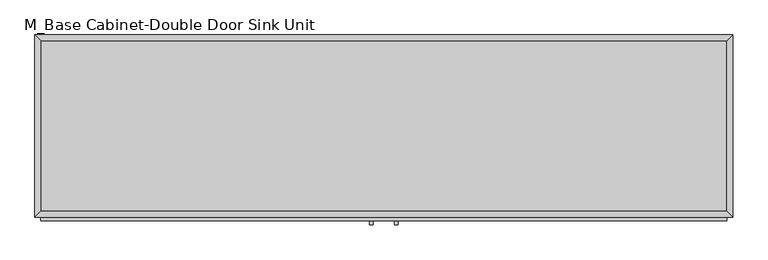
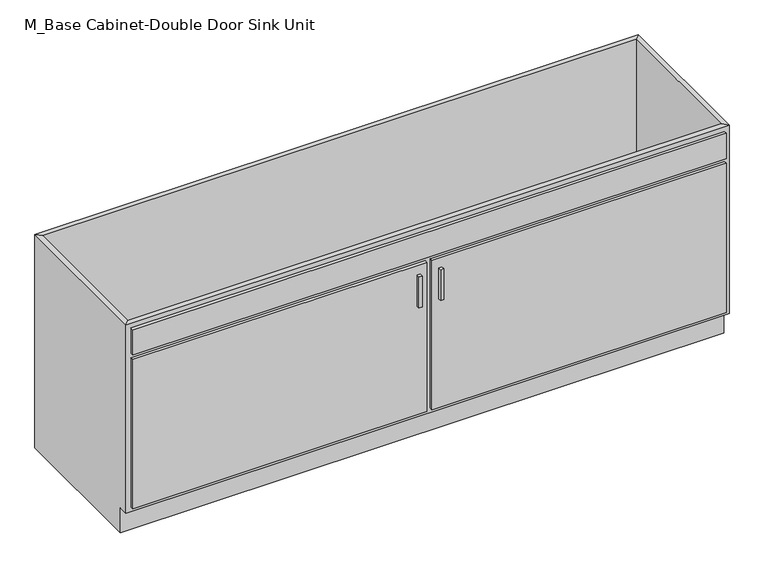
"""IFC4 building model written with IfcOpenShell, lengths in millimetres: furniture geometry, M_Base Cabinet-Double Door Sink Unit : UEBLEE."""

import ifcopenshell
import ifcopenshell.guid

model = None  # the IFC model being written
_history = None  # IfcOwnerHistory: only IFC2X3 demands one
_inside = {}  # id of a spatial element -> (the spatial element, [elements in it])
_under = {}  # id of a project, library or spatial element -> (it, [spatial elements below it])
_declared = {}  # id of a project -> (the project, [libraries it declares])
_typed = {}  # id of a type object -> (the type object, [elements of that type])
_made_of = {}  # id of a material, layer set ... -> (it, [elements and type objects made of it])


def new_model(schema):
    """Start an empty IFC model of exactly this schema.

    Asked for "IFC4X3", IfcOpenShell would pick the latest addendum, in which some entities
    have other attributes; the version numbers below select the first issue.
    IFC2X3 requires an IfcOwnerHistory on every rooted entity: one is made here for all.
    """
    global model, _history
    if schema == "IFC4X3":
        model = ifcopenshell.file(schema_version=(4, 3, 0, 0))
    else:
        model = ifcopenshell.file(schema=schema)
    _inside.clear()
    _under.clear()
    _declared.clear()
    _typed.clear()
    _made_of.clear()
    _history = None
    if model.schema == "IFC2X3":
        org = make("IfcOrganization", Name="unknown")
        user = make(
            "IfcPersonAndOrganization",
            ThePerson=make("IfcPerson", FamilyName="unknown"),
            TheOrganization=org,
        )
        app = make(
            "IfcApplication",
            ApplicationDeveloper=org,
            Version="unknown",
            ApplicationFullName="unknown",
            ApplicationIdentifier="unknown",
        )
        _history = make(
            "IfcOwnerHistory",
            OwningUser=user,
            OwningApplication=app,
            ChangeAction="ADDED",
            CreationDate=0,
        )
    return model


def make(cls, **values):
    """One entity of the class cls with the attributes given. An attribute that is None is left unset."""
    return model.create_entity(
        cls, **{name: value for name, value in values.items() if value is not None}
    )


def rooted(cls, **values):
    """An entity with a GlobalId (a new one), such as an element, a storey or a relation."""
    return make(cls, GlobalId=ifcopenshell.guid.new(), OwnerHistory=_history, **values)


def si_unit(unit_type, name, prefix=None):
    """IfcSIUnit, for example si_unit("LENGTHUNIT", "METRE", prefix="MILLI")."""
    return make("IfcSIUnit", UnitType=unit_type, Prefix=prefix, Name=name)


def assignment(units):
    """IfcUnitAssignment: the units of a project."""
    return None if units is None else make("IfcUnitAssignment", Units=units)


def point(xyz):
    """IfcCartesianPoint."""
    return None if xyz is None else make("IfcCartesianPoint", Coordinates=xyz)


def direction(xyz):
    """IfcDirection."""
    return None if xyz is None else make("IfcDirection", DirectionRatios=xyz)


def frame(location, z_axis=None, x_axis=None):
    """IfcAxis2Placement3D, a coordinate frame: its origin and axes. An axis left out is left unset."""
    return make(
        "IfcAxis2Placement3D",
        Location=point(location),
        Axis=direction(z_axis),
        RefDirection=direction(x_axis),
    )


def origin():
    """The frame at (0, 0, 0) with its axes left unset."""
    return frame((0.0, 0.0, 0.0))


def place(relative_to, where):
    """IfcLocalPlacement: puts the frame where relative to a parent placement (None: the world)."""
    return make(
        "IfcLocalPlacement", PlacementRelTo=relative_to, RelativePlacement=where
    )


def context(
    kind, dimensions, precision=None, world=None, true_north=None, identifier=None
):
    """IfcGeometricRepresentationContext, for example the 3D "Model" context."""
    return make(
        "IfcGeometricRepresentationContext",
        ContextIdentifier=identifier,
        ContextType=kind,
        CoordinateSpaceDimension=dimensions,
        Precision=precision,
        WorldCoordinateSystem=world,
        TrueNorth=true_north,
    )


def project(units=None, contexts=None):
    """IfcProject with its units and contexts."""
    return rooted(
        "IfcProject",
        Name="project",
        RepresentationContexts=contexts,
        UnitsInContext=assignment(units),
    )


def spatial(cls, under=None, at=None, **own):
    """A site, building, storey or space (cls), placed at a placement, below another one or the project."""
    s = rooted(cls, ObjectPlacement=at, **own)
    if under is not None:
        _under.setdefault(under.id(), (under, []))[1].append(s)
    return s


def polyline(points):
    """IfcPolyline through the points."""
    return make("IfcPolyline", Points=[point(p) for p in points])


def outline(outer, holes=None, kind="AREA"):
    """IfcArbitraryClosedProfileDef: a profile drawn as a closed curve; with holes, ...WithVoids."""
    if holes is None:
        return make("IfcArbitraryClosedProfileDef", ProfileType=kind, OuterCurve=outer)
    return make(
        "IfcArbitraryProfileDefWithVoids",
        ProfileType=kind,
        OuterCurve=outer,
        InnerCurves=holes,
    )


def extrude(swept, where, along, depth):
    """IfcExtrudedAreaSolid: the profile swept, set in the frame where, extruded along a direction by depth."""
    return make(
        "IfcExtrudedAreaSolid",
        SweptArea=swept,
        Position=where,
        ExtrudedDirection=direction(along),
        Depth=depth,
    )


def faces_of(points, faces, orient=None, outer=None):
    """IfcFace entities. A face is a list of loops; a loop is a list of indices into points, from 0.

    orient and outer hold one flag for each loop. By default every Orientation is true, the
    first loop of a face is its IfcFaceOuterBound and the others are IfcFaceBound.
    """
    made = []
    for i, loops in enumerate(faces):
        bounds = []
        for j, loop in enumerate(loops):
            is_outer = j == 0 if outer is None else outer[i][j]
            bounds.append(
                make(
                    "IfcFaceOuterBound" if is_outer else "IfcFaceBound",
                    Bound=make("IfcPolyLoop", Polygon=[points[k] for k in loop]),
                    Orientation=True if orient is None else orient[i][j],
                )
            )
        made.append(make("IfcFace", Bounds=bounds))
    return made


def faceted_brep(points, faces, orient=None, outer=None, voids=None):
    """IfcFacetedBrep: a solid bounded by flat faces; with voids (closed shells), ...WithVoids."""
    shared = [point(p) for p in points]
    hull = make("IfcClosedShell", CfsFaces=faces_of(shared, faces, orient, outer))
    if voids is None:
        return make("IfcFacetedBrep", Outer=hull)
    return make(
        "IfcFacetedBrepWithVoids",
        Outer=hull,
        Voids=[
            make(cls, CfsFaces=faces_of(shared, fs, o, b)) for cls, fs, o, b in voids
        ],
    )


def shape(context_of_items, identifier, shape_type, items):
    """IfcShapeRepresentation: the items that make up one representation, for example the "Body"."""
    return make(
        "IfcShapeRepresentation",
        ContextOfItems=context_of_items,
        RepresentationIdentifier=identifier,
        RepresentationType=shape_type,
        Items=items,
    )


def source(mapping_origin, context_of_items, identifier, shape_type, items):
    """IfcRepresentationMap: a shape defined once, which mapped items show again and again."""
    return make(
        "IfcRepresentationMap",
        MappingOrigin=mapping_origin,
        MappedRepresentation=shape(context_of_items, identifier, shape_type, items),
    )


def transform(
    local_origin,
    x_axis=None,
    y_axis=None,
    z_axis=None,
    scale=None,
    scale2=None,
    scale3=None,
    uniform=True,
):
    """IfcCartesianTransformationOperator3D, or its non-uniform kind. x_axis, y_axis, z_axis: its Axis1, 2, 3."""
    if uniform:
        return make(
            "IfcCartesianTransformationOperator3D",
            Axis1=direction(x_axis),
            Axis2=direction(y_axis),
            LocalOrigin=point(local_origin),
            Scale=scale,
            Axis3=direction(z_axis),
        )
    return make(
        "IfcCartesianTransformationOperator3DnonUniform",
        Axis1=direction(x_axis),
        Axis2=direction(y_axis),
        LocalOrigin=point(local_origin),
        Scale=scale,
        Axis3=direction(z_axis),
        Scale2=scale2,
        Scale3=scale3,
    )


def mapped(mapping_source, mapping_target):
    """IfcMappedItem: shows the shape of a source again, moved by a transform."""
    return make(
        "IfcMappedItem", MappingSource=mapping_source, MappingTarget=mapping_target
    )


def made_of(thing, what):
    """Note that an element or type object is made of a material, layer set ...; save() writes the relation."""
    if what is not None:
        _made_of.setdefault(what.id(), (what, []))[1].append(thing)
    return thing


def element(
    cls,
    number,
    at=None,
    inside=None,
    cuts=None,
    type_object=None,
    material=None,
    context=None,
    identifier="Body",
    shape_type=None,
    held_by="IfcProductDefinitionShape",
    body=None,
    shapes=None,
    **own,
):
    """One element of the class cls, such as IfcWall. Its Tag is "e" and its number.

    at: its placement. inside: the storey or other place that contains it. cuts: it is an
    opening in that element (IfcRelVoidsElement). A single representation is given by context,
    identifier, shape_type and body (its items); several are given by shapes. held_by: the class
    of the entity that holds the representations. save() writes the other relations.
    """
    e = rooted(cls, Tag="e%d" % number, ObjectPlacement=at, **own)
    if body is not None:
        shapes = [shape(context, identifier, shape_type, body)]
    if shapes is not None:
        e.Representation = make(held_by, Representations=shapes)
    if inside is not None:
        _inside.setdefault(inside.id(), (inside, []))[1].append(e)
    if cuts is not None:
        rooted(
            "IfcRelVoidsElement", RelatingBuildingElement=cuts, RelatedOpeningElement=e
        )
    if type_object is not None:
        _typed.setdefault(type_object.id(), (type_object, []))[1].append(e)
    return made_of(e, material)


def aggregate(whole, parts):
    """IfcRelAggregates: a whole, such as a stair, and the parts it consists of."""
    return rooted("IfcRelAggregates", RelatingObject=whole, RelatedObjects=parts)


def save(model, path):
    """Write the relations noted so far, then the file.

    IfcRelAggregates (storeys below a building ...), IfcRelContainedInSpatialStructure (elements
    in a storey), IfcRelDefinesByType, IfcRelAssociatesMaterial and IfcRelDeclares: one each for
    every whole, place, type object, material and project.
    """
    for whole, parts in _under.values():
        aggregate(whole, parts)
    for where, things in _inside.values():
        rooted(
            "IfcRelContainedInSpatialStructure",
            RelatedElements=things,
            RelatingStructure=where,
        )
    for kind, things in _typed.values():
        rooted("IfcRelDefinesByType", RelatedObjects=things, RelatingType=kind)
    for what, things in _made_of.values():
        rooted("IfcRelAssociatesMaterial", RelatedObjects=things, RelatingMaterial=what)
    for by, libraries in _declared.values():
        rooted("IfcRelDeclares", RelatingContext=by, RelatedDefinitions=libraries)
    model.write(path)


def m_base_cabinet_double_door_sink_unit_48243878(model_context):
    return source(origin(), model_context, "Body", "SolidModel", [
        faceted_brep([(1149.6877049, -580.95, 860.0), (1149.6877049, -580.95, 100.0), (-1112.2122951, -580.95, 100.0), (-1112.2122951, -580.95, 860.0), (-1131.2622951, -600.0, 860.0), (1168.7377049, -600.0, 860.0), (-1131.2622951, -600.0, 100.0), (1168.7377049, -600.0, 100.0), (-1112.2122951, -565.0, 100.0), (-1112.2122951, -19.05, 100.0), (-1112.2122951, -19.05, 860.0), (-1131.2622951, 0.0, 860.0), (-1131.2622951, 0.0, 0.0), (-1131.2622951, -565.0, 0.0), (-1131.2622951, -565.0, 100.0), (1149.6877049, -19.05, 100.0), (1149.6877049, -19.05, 860.0), (1168.7377049, 0.0, 860.0), (1168.7377049, 0.0, 0.0), (1149.6877049, -565.0, 100.0), (1168.7377049, -565.0, 100.0), (1168.7377049, -565.0, 0.0)], [[[0, 1, 2, 3]], [[0, 3, 4, 5]], [[5, 4, 6, 7]], [[2, 1, 7, 6]], [[3, 2, 8, 9, 10]], [[4, 3, 10, 11]], [[6, 4, 11, 12, 13, 14]], [[2, 6, 14, 8]], [[10, 9, 15, 16]], [[11, 10, 16, 17]], [[12, 11, 17, 18]], [[1, 0, 16, 15, 19]], [[0, 5, 17, 16]], [[5, 7, 20, 21, 18, 17]], [[7, 1, 19, 20]], [[8, 19, 15, 9]], [[18, 21, 13, 12]], [[13, 21, 20, 19, 8, 14]]]),
        extrude(outline(polyline([(-16.1872951, -625.4), (-28.8872951, -625.4), (-28.8872951, -612.7), (-16.1872951, -612.7), (-16.1872951, -625.4)])), frame((0.0, 0.0, 557.469895), z_axis=(0.0, 0.0, 1.0), x_axis=(1.0, 0.0, 0.0)), (0.0, 0.0, 1.0), 124.730105),
        extrude(outline(polyline([(66.3627049, -625.4), (53.6627049, -625.4), (53.6627049, -612.7), (66.3627049, -612.7), (66.3627049, -625.4)])), frame((0.0, 0.0, 557.469895), z_axis=(0.0, 0.0, 1.0), x_axis=(1.0, 0.0, 0.0)), (0.0, 0.0, 1.0), 124.730105),
        extrude(outline(polyline([(9.2127049, -612.7), (-1112.2122951, -612.7), (-1112.2122951, -600.0), (9.2127049, -600.0), (9.2127049, -612.7)])), frame((0.0, 0.0, 119.05), z_axis=(0.0, 0.0, 1.0), x_axis=(1.0, 0.0, 0.0)), (0.0, 0.0, 1.0), 601.25),
        extrude(outline(polyline([(1149.6877049, -612.7), (28.2627049, -612.7), (28.2627049, -600.0), (1149.6877049, -600.0), (1149.6877049, -612.7)])), frame((0.0, 0.0, 119.05), z_axis=(0.0, 0.0, 1.0), x_axis=(1.0, 0.0, 0.0)), (0.0, 0.0, 1.0), 601.25),
        extrude(outline(polyline([(1149.6877049, -612.7), (-1112.2122951, -612.7), (-1112.2122951, -600.0), (1149.6877049, -600.0), (1149.6877049, -612.7)])), frame((0.0, 0.0, 739.35), z_axis=(0.0, 0.0, 1.0), x_axis=(1.0, 0.0, 0.0)), (0.0, 0.0, 1.0), 101.6),
        extrude(outline(polyline([(1149.6877049, -19.05), (1149.6877049, -580.95), (-1112.2122951, -580.95), (-1112.2122951, -19.05), (1149.6877049, -19.05)])), frame((0.0, 0.0, 100.0), z_axis=(0.0, 0.0, 1.0), x_axis=(1.0, 0.0, 0.0)), (0.0, 0.0, 1.0), 19.05),
    ])


if __name__ == "__main__":
    model = new_model("IFC4")
    model_context = context("Model", 3, world=origin())
    ifc_project = project(units=[si_unit("LENGTHUNIT", "METRE", prefix="MILLI")], contexts=[model_context])
    site = spatial("IfcSite", under=ifc_project)
    building = spatial("IfcBuilding", under=site)
    placement = place(None, origin())
    m_base_cabinet_double_door_sink_unit_shape = m_base_cabinet_double_door_sink_unit_48243878(model_context)
    element("IfcFurniture", 1, ObjectType="M_Base Cabinet-Double Door Sink Unit : UEBLEE", at=placement, inside=building, context=model_context, shape_type="MappedRepresentation", body=[
        mapped(m_base_cabinet_double_door_sink_unit_shape, transform((0.0, 0.0, 0.0), x_axis=(1.0, 0.0, 0.0), y_axis=(0.0, 1.0, 0.0), z_axis=(0.0, 0.0, 1.0))),
    ])
    save(model, "model.ifc")

# Revit data of these elements
# Type "M_Base Cabinet-Double Door Sink Unit : UEBLEE"
#   Depth = 0.60 m
#   Height = 0.86 m
#   Plinth Depth = 0.035 m
#   Plinth Height = 0.10 m
#   Width = 2.30 m
#   Cabinet Material = none
#   Door/Drawer Material = none
#   Handle Material = Cabinets - Handles
#   Default Elevation = 0
# Element 1 (IfcFurniture, "M_Base Cabinet-Double Door Sink Unit : UEBLEE")
#   Materials on its faces: "Cabinets", "Cabinets - Handles"
# Materials
#   "Cabinets - Handles": class "Metal", colour RGB 57 57 57, transparency 0
#   "Cabinets": class "Miscellaneous", colour RGB 249 249 249, transparency 0
